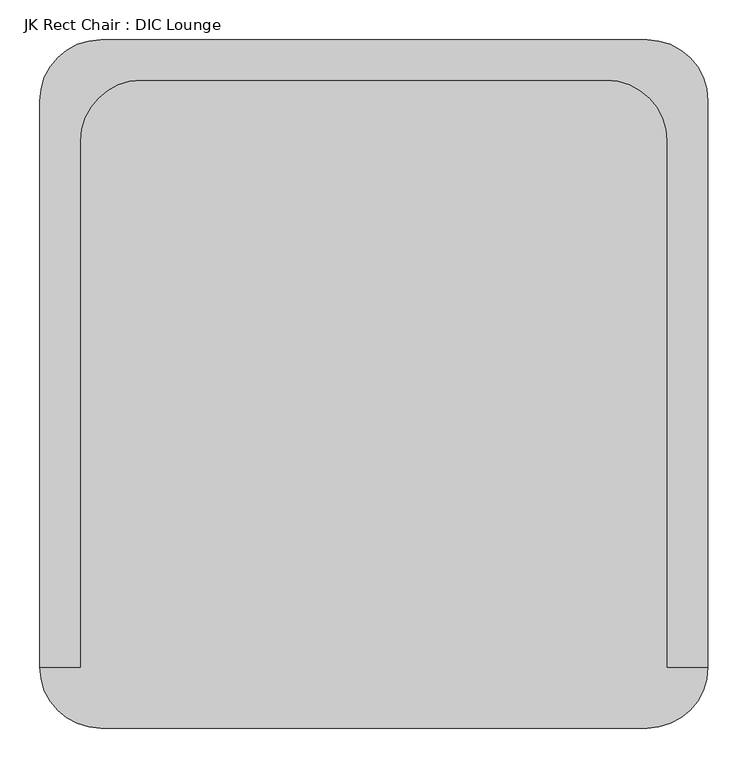
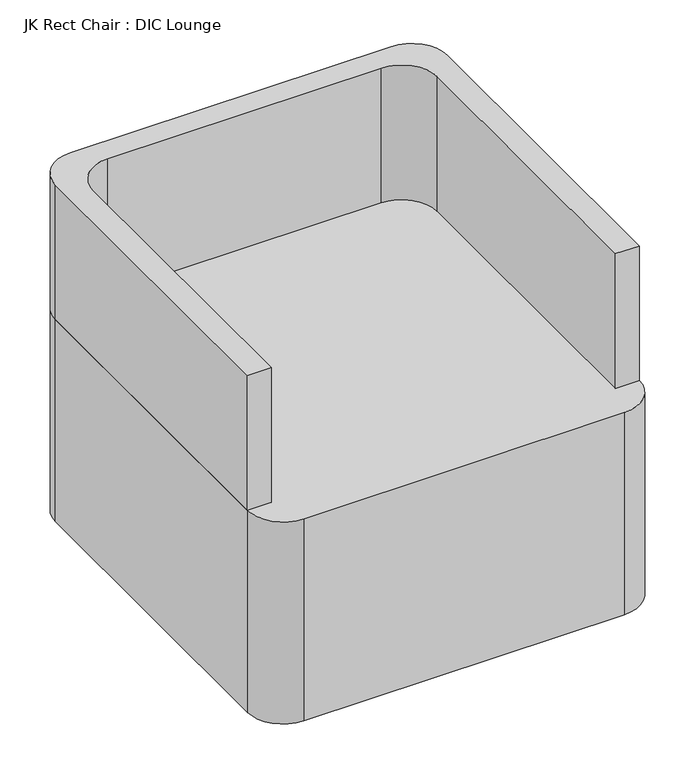
"""IFC4 building model written with IfcOpenShell, lengths in millimetres: furniture geometry, JK Rect Chair : DIC Lounge."""

from ifc_helpers import new_model, si_unit, point, frame, frame_2d, origin, origin_with_axes, place, context, project, spatial, polyline, circle_curve, trimmed, segment, composite_curve, outline, extrude, source, transform, mapped, element, save


def jk_rect_chair_dic_lounge_4de9fba9(model_context):
    return source(origin(), model_context, "Body", "SweptSolid", [
        extrude(outline(composite_curve([segment(polyline([(-430.2426335, -322.0544704), (-481.0426335, -322.0544704), (-481.0426335, 389.1455296)]), True, "CONTINUOUS"), segment(trimmed(circle_curve(frame_2d((-404.8426335, 389.1455296)), 76.2), [point((-481.0426335, 389.1455296))], [point((-404.8426335, 465.3455296))], False, "CARTESIAN"), True, "CONTINUOUS"), segment(polyline([(-404.8426335, 465.3455296), (280.9573665, 465.3455296)]), True, "CONTINUOUS"), segment(trimmed(circle_curve(frame_2d((280.9573665, 389.1455296)), 76.2), [point((280.9573665, 465.3455296))], [point((357.1573665, 389.1455296))], False, "CARTESIAN"), True, "CONTINUOUS"), segment(polyline([(357.1573665, 389.1455296), (357.1573665, -322.0544704), (306.3573665, -322.0544704), (306.3573665, 338.3455296)]), True, "CONTINUOUS"), segment(trimmed(circle_curve(frame_2d((230.1573665, 338.3455296)), 76.2), [point((306.3573665, 338.3455296))], [point((230.1573665, 414.5455296))], True, "CARTESIAN"), True, "CONTINUOUS"), segment(polyline([(230.1573665, 414.5455296), (-354.0426335, 414.5455296)]), True, "CONTINUOUS"), segment(trimmed(circle_curve(frame_2d((-354.0426335, 338.3455296)), 76.2), [point((-354.0426335, 414.5455296))], [point((-430.2426335, 338.3455296))], True, "CARTESIAN"), True, "CONTINUOUS"), segment(polyline([(-430.2426335, 338.3455296), (-430.2426335, -322.0544704)]), True, "CONTINUOUS")], self_intersect=False)), frame((0.0, 0.0, 457.2), z_axis=(0.0, 0.0, 1.0), x_axis=(1.0, 0.0, 0.0)), (0.0, 0.0, 1.0), 304.8),
        extrude(outline(composite_curve([segment(trimmed(circle_curve(frame_2d((-404.8426335, 389.1455296)), 76.2), [point((-481.0426335, 389.1455296))], [point((-404.8426335, 465.3455296))], False, "CARTESIAN"), True, "CONTINUOUS"), segment(polyline([(-404.8426335, 465.3455296), (280.9573665, 465.3455296)]), True, "CONTINUOUS"), segment(trimmed(circle_curve(frame_2d((280.9573665, 389.1455296)), 76.2), [point((280.9573665, 465.3455296))], [point((357.1573665, 389.1455296))], False, "CARTESIAN"), True, "CONTINUOUS"), segment(polyline([(357.1573665, 389.1455296), (357.1573665, -322.0544704)]), True, "CONTINUOUS"), segment(trimmed(circle_curve(frame_2d((280.9573665, -322.0544704)), 76.2), [point((357.1573665, -322.0544704))], [point((280.9573665, -398.2544704))], False, "CARTESIAN"), True, "CONTINUOUS"), segment(polyline([(280.9573665, -398.2544704), (-404.8426335, -398.2544704)]), True, "CONTINUOUS"), segment(trimmed(circle_curve(frame_2d((-404.8426335, -322.0544704)), 76.2), [point((-404.8426335, -398.2544704))], [point((-481.0426335, -322.0544704))], False, "CARTESIAN"), True, "CONTINUOUS"), segment(polyline([(-481.0426335, -322.0544704), (-481.0426335, 389.1455296)]), True, "CONTINUOUS")], self_intersect=False)), origin_with_axes(), (0.0, 0.0, 1.0), 457.2),
    ])


if __name__ == "__main__":
    model = new_model("IFC4")
    model_context = context("Model", 3, world=origin())
    ifc_project = project(units=[si_unit("LENGTHUNIT", "METRE", prefix="MILLI")], contexts=[model_context])
    site = spatial("IfcSite", under=ifc_project)
    building = spatial("IfcBuilding", under=site)
    placement = place(None, origin())
    jk_rect_chair_dic_lounge_shape = jk_rect_chair_dic_lounge_4de9fba9(model_context)
    element("IfcFurniture", 1, ObjectType="JK Rect Chair : DIC Lounge", at=placement, inside=building, context=model_context, shape_type="MappedRepresentation", body=[
        mapped(jk_rect_chair_dic_lounge_shape, transform((0.0, 0.0, 0.0), x_axis=(1.0, 0.0, 0.0), y_axis=(0.0, 1.0, 0.0), z_axis=(0.0, 0.0, 1.0))),
    ])
    save(model, "model.ifc")

# Revit data of these elements
# Type "JK Rect Chair : DIC Lounge"
#   Width = 2' - 9"
#   Seat Height = 1' - 6"
#   Depth = 2' - 10"
#   Corner Radius = 0' - 3"
#   Back Height = 2' - 6"
#   Status [instance default] = none
#   Default Elevation = 0
